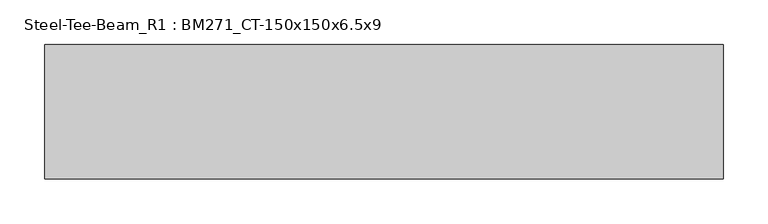
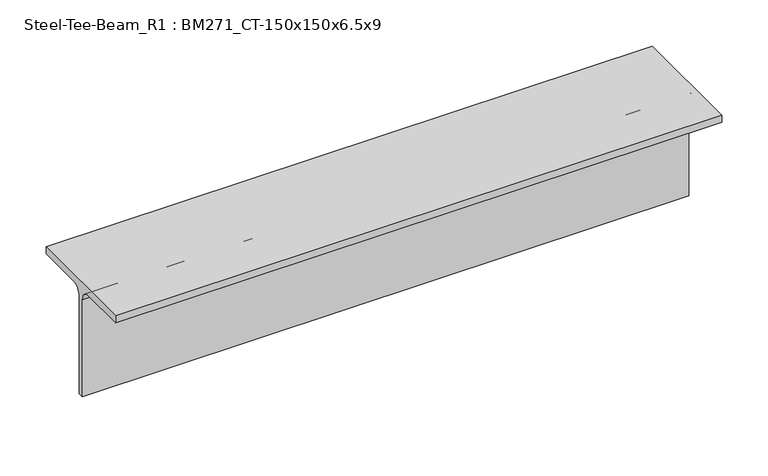
"""IFC4 building model written with IfcOpenShell, lengths in millimetres: member geometry, Steel-Tee-Beam_R1 : BM271_CT-150x150x6.5x9."""

from ifc_helpers import new_model, si_unit, point, frame, frame_2d, origin, place, context, project, spatial, polyline, circle_curve, trimmed, segment, composite_curve, outline, extrude, source, transform, mapped, element, save


def steel_tee_beam_r1_bm271_ct_150x150x6_5x9_4ba03e4c(model_context):
    return source(origin(), model_context, "Body", "SweptSolid", [
        extrude(outline(composite_curve([segment(polyline([(-75.0, 75.0), (75.0, 75.0), (75.0, 66.0), (16.25, 66.0)]), True, "CONTINUOUS"), segment(trimmed(circle_curve(frame_2d((16.25, 53.0)), 13.0), [point((16.25, 66.0))], [point((3.25, 53.0))], True, "CARTESIAN"), True, "CONTINUOUS"), segment(polyline([(3.25, 53.0), (3.25, -75.0), (-3.25, -75.0), (-3.25, 53.0)]), True, "CONTINUOUS"), segment(trimmed(circle_curve(frame_2d((-16.25, 53.0)), 13.0), [point((-3.25, 53.0))], [point((-16.25, 66.0))], True, "CARTESIAN"), True, "CONTINUOUS"), segment(polyline([(-16.25, 66.0), (-75.0, 66.0), (-75.0, 75.0)]), True, "CONTINUOUS")], self_intersect=False)), frame((-403.3208745, 0.0, 0.0), z_axis=(1.0, 0.0, 0.0), x_axis=(0.0, 1.0, 0.0)), (0.0, 0.0, 1.0), 756.4352524),
    ])


if __name__ == "__main__":
    model = new_model("IFC4")
    model_context = context("Model", 3, world=origin())
    ifc_project = project(units=[si_unit("LENGTHUNIT", "METRE", prefix="MILLI")], contexts=[model_context])
    site = spatial("IfcSite", under=ifc_project)
    building = spatial("IfcBuilding", under=site)
    placement = place(None, origin())
    steel_tee_beam_r1_bm271_ct_150x150x6_5x9_shape = steel_tee_beam_r1_bm271_ct_150x150x6_5x9_4ba03e4c(model_context)
    element("IfcMember", 1, ObjectType="Steel-Tee-Beam_R1 : BM271_CT-150x150x6.5x9", at=placement, inside=building, context=model_context, shape_type="MappedRepresentation", body=[
        mapped(steel_tee_beam_r1_bm271_ct_150x150x6_5x9_shape, transform((0.0, 0.0, 0.0), x_axis=(1.0, 0.0, 0.0), y_axis=(0.0, 1.0, 0.0), z_axis=(0.0, 0.0, 1.0))),
    ])
    save(model, "model.ifc")

# Revit data of these elements
# Type "Steel-Tee-Beam_R1 : BM271_CT-150x150x6.5x9"
#   Keynote = "CT-150x150x6.5x9"
#   Surface Area = 0.588841 m²/m
#   Section Area = 23.3904 cm²
#   Mass per Unit Length = 18.3614 kg/m
#   Length [instance default] = 1.5240 m
#   bf = 0.1500 m
#   d = 0.1500 m
#   k = 0.0220 m
#   r = 0.0130 m
#   tf = 0.0090 m
#   tw = 0.0065 m
#   hec_material4 [instance default] = none
#   hec_material3 [instance default] = none
#   hec_material2 [instance default] = none
#   hec_material1 [instance default] = none
#   Structural Material [instance default] = Steel, 45-345
#   Assembly Code = ""
# Element 1 (IfcMember, "Steel-Tee-Beam_R1 : BM271_CT-150x150x6.5x9")
#   Structural Material = none
# Materials
#   "Steel, 45-345": class "Metal", colour RGB 189 187 185, transparency 0, Description = "Steel 345 MPa", Cost = 0
